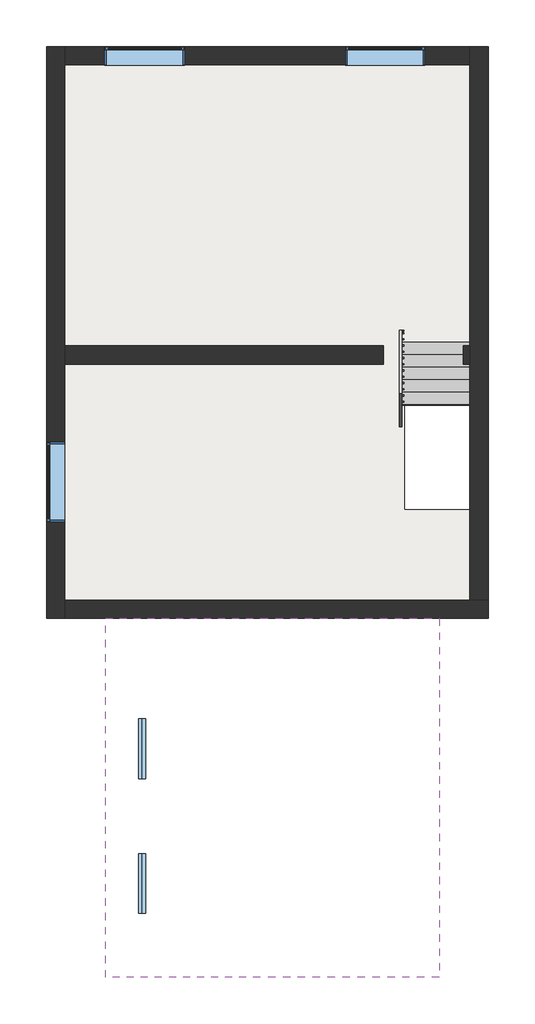
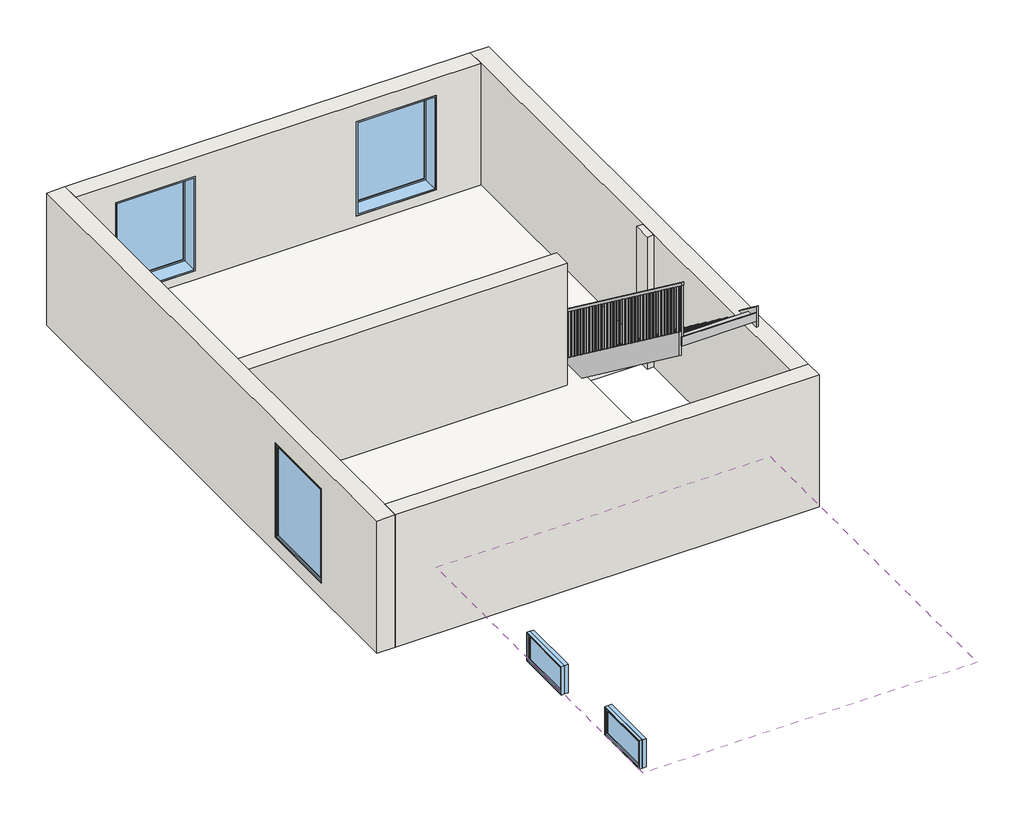
# One storey: 5 walls, 5 windows, 2 members, 1 railing, 1 roof, 1 slab, 1 stair flight.
"""IFC4 building model written with IfcOpenShell, lengths in millimetres."""

import ifcopenshell
import ifcopenshell.guid

model = None  # the IFC model being written
_history = None  # IfcOwnerHistory: only IFC2X3 demands one
_inside = {}  # id of a spatial element -> (the spatial element, [elements in it])
_under = {}  # id of a project, library or spatial element -> (it, [spatial elements below it])
_declared = {}  # id of a project -> (the project, [libraries it declares])
_typed = {}  # id of a type object -> (the type object, [elements of that type])
_made_of = {}  # id of a material, layer set ... -> (it, [elements and type objects made of it])


def new_model(schema):
    """Start an empty IFC model of exactly this schema.

    Asked for "IFC4X3", IfcOpenShell would pick the latest addendum, in which some entities
    have other attributes; the version numbers below select the first issue.
    IFC2X3 requires an IfcOwnerHistory on every rooted entity: one is made here for all.
    """
    global model, _history
    if schema == "IFC4X3":
        model = ifcopenshell.file(schema_version=(4, 3, 0, 0))
    else:
        model = ifcopenshell.file(schema=schema)
    _inside.clear()
    _under.clear()
    _declared.clear()
    _typed.clear()
    _made_of.clear()
    _history = None
    if model.schema == "IFC2X3":
        org = make("IfcOrganization", Name="unknown")
        user = make(
            "IfcPersonAndOrganization",
            ThePerson=make("IfcPerson", FamilyName="unknown"),
            TheOrganization=org,
        )
        app = make(
            "IfcApplication",
            ApplicationDeveloper=org,
            Version="unknown",
            ApplicationFullName="unknown",
            ApplicationIdentifier="unknown",
        )
        _history = make(
            "IfcOwnerHistory",
            OwningUser=user,
            OwningApplication=app,
            ChangeAction="ADDED",
            CreationDate=0,
        )
    return model


def make(cls, **values):
    """One entity of the class cls with the attributes given. An attribute that is None is left unset."""
    return model.create_entity(
        cls, **{name: value for name, value in values.items() if value is not None}
    )


def rooted(cls, **values):
    """An entity with a GlobalId (a new one), such as an element, a storey or a relation."""
    return make(cls, GlobalId=ifcopenshell.guid.new(), OwnerHistory=_history, **values)


def si_unit(unit_type, name, prefix=None):
    """IfcSIUnit, for example si_unit("LENGTHUNIT", "METRE", prefix="MILLI")."""
    return make("IfcSIUnit", UnitType=unit_type, Prefix=prefix, Name=name)


def assignment(units):
    """IfcUnitAssignment: the units of a project."""
    return None if units is None else make("IfcUnitAssignment", Units=units)


def point(xyz):
    """IfcCartesianPoint."""
    return None if xyz is None else make("IfcCartesianPoint", Coordinates=xyz)


def direction(xyz):
    """IfcDirection."""
    return None if xyz is None else make("IfcDirection", DirectionRatios=xyz)


def frame(location, z_axis=None, x_axis=None):
    """IfcAxis2Placement3D, a coordinate frame: its origin and axes. An axis left out is left unset."""
    return make(
        "IfcAxis2Placement3D",
        Location=point(location),
        Axis=direction(z_axis),
        RefDirection=direction(x_axis),
    )


def origin():
    """The frame at (0, 0, 0) with its axes left unset."""
    return frame((0.0, 0.0, 0.0))


def place(relative_to, where):
    """IfcLocalPlacement: puts the frame where relative to a parent placement (None: the world)."""
    return make(
        "IfcLocalPlacement", PlacementRelTo=relative_to, RelativePlacement=where
    )


def context(
    kind, dimensions, precision=None, world=None, true_north=None, identifier=None
):
    """IfcGeometricRepresentationContext, for example the 3D "Model" context."""
    return make(
        "IfcGeometricRepresentationContext",
        ContextIdentifier=identifier,
        ContextType=kind,
        CoordinateSpaceDimension=dimensions,
        Precision=precision,
        WorldCoordinateSystem=world,
        TrueNorth=true_north,
    )


def project(units=None, contexts=None):
    """IfcProject with its units and contexts."""
    return rooted(
        "IfcProject",
        Name="project",
        RepresentationContexts=contexts,
        UnitsInContext=assignment(units),
    )


def spatial(cls, under=None, at=None, **own):
    """A site, building, storey or space (cls), placed at a placement, below another one or the project."""
    s = rooted(cls, ObjectPlacement=at, **own)
    if under is not None:
        _under.setdefault(under.id(), (under, []))[1].append(s)
    return s


def polyline(points):
    """IfcPolyline through the points."""
    return make("IfcPolyline", Points=[point(p) for p in points])


def outline(outer, holes=None, kind="AREA"):
    """IfcArbitraryClosedProfileDef: a profile drawn as a closed curve; with holes, ...WithVoids."""
    if holes is None:
        return make("IfcArbitraryClosedProfileDef", ProfileType=kind, OuterCurve=outer)
    return make(
        "IfcArbitraryProfileDefWithVoids",
        ProfileType=kind,
        OuterCurve=outer,
        InnerCurves=holes,
    )


def extrude(swept, where, along, depth):
    """IfcExtrudedAreaSolid: the profile swept, set in the frame where, extruded along a direction by depth."""
    return make(
        "IfcExtrudedAreaSolid",
        SweptArea=swept,
        Position=where,
        ExtrudedDirection=direction(along),
        Depth=depth,
    )


def faces_of(points, faces, orient=None, outer=None):
    """IfcFace entities. A face is a list of loops; a loop is a list of indices into points, from 0.

    orient and outer hold one flag for each loop. By default every Orientation is true, the
    first loop of a face is its IfcFaceOuterBound and the others are IfcFaceBound.
    """
    made = []
    for i, loops in enumerate(faces):
        bounds = []
        for j, loop in enumerate(loops):
            is_outer = j == 0 if outer is None else outer[i][j]
            bounds.append(
                make(
                    "IfcFaceOuterBound" if is_outer else "IfcFaceBound",
                    Bound=make("IfcPolyLoop", Polygon=[points[k] for k in loop]),
                    Orientation=True if orient is None else orient[i][j],
                )
            )
        made.append(make("IfcFace", Bounds=bounds))
    return made


def faceted_brep(points, faces, orient=None, outer=None, voids=None):
    """IfcFacetedBrep: a solid bounded by flat faces; with voids (closed shells), ...WithVoids."""
    shared = [point(p) for p in points]
    hull = make("IfcClosedShell", CfsFaces=faces_of(shared, faces, orient, outer))
    if voids is None:
        return make("IfcFacetedBrep", Outer=hull)
    return make(
        "IfcFacetedBrepWithVoids",
        Outer=hull,
        Voids=[
            make(cls, CfsFaces=faces_of(shared, fs, o, b)) for cls, fs, o, b in voids
        ],
    )


def shape(context_of_items, identifier, shape_type, items):
    """IfcShapeRepresentation: the items that make up one representation, for example the "Body"."""
    return make(
        "IfcShapeRepresentation",
        ContextOfItems=context_of_items,
        RepresentationIdentifier=identifier,
        RepresentationType=shape_type,
        Items=items,
    )


def source(mapping_origin, context_of_items, identifier, shape_type, items):
    """IfcRepresentationMap: a shape defined once, which mapped items show again and again."""
    return make(
        "IfcRepresentationMap",
        MappingOrigin=mapping_origin,
        MappedRepresentation=shape(context_of_items, identifier, shape_type, items),
    )


def transform(
    local_origin,
    x_axis=None,
    y_axis=None,
    z_axis=None,
    scale=None,
    scale2=None,
    scale3=None,
    uniform=True,
):
    """IfcCartesianTransformationOperator3D, or its non-uniform kind. x_axis, y_axis, z_axis: its Axis1, 2, 3."""
    if uniform:
        return make(
            "IfcCartesianTransformationOperator3D",
            Axis1=direction(x_axis),
            Axis2=direction(y_axis),
            LocalOrigin=point(local_origin),
            Scale=scale,
            Axis3=direction(z_axis),
        )
    return make(
        "IfcCartesianTransformationOperator3DnonUniform",
        Axis1=direction(x_axis),
        Axis2=direction(y_axis),
        LocalOrigin=point(local_origin),
        Scale=scale,
        Axis3=direction(z_axis),
        Scale2=scale2,
        Scale3=scale3,
    )


def mapped(mapping_source, mapping_target):
    """IfcMappedItem: shows the shape of a source again, moved by a transform."""
    return make(
        "IfcMappedItem", MappingSource=mapping_source, MappingTarget=mapping_target
    )


def made_of(thing, what):
    """Note that an element or type object is made of a material, layer set ...; save() writes the relation."""
    if what is not None:
        _made_of.setdefault(what.id(), (what, []))[1].append(thing)
    return thing


def element(
    cls,
    number,
    at=None,
    inside=None,
    cuts=None,
    type_object=None,
    material=None,
    context=None,
    identifier="Body",
    shape_type=None,
    held_by="IfcProductDefinitionShape",
    body=None,
    shapes=None,
    **own,
):
    """One element of the class cls, such as IfcWall. Its Tag is "e" and its number.

    at: its placement. inside: the storey or other place that contains it. cuts: it is an
    opening in that element (IfcRelVoidsElement). A single representation is given by context,
    identifier, shape_type and body (its items); several are given by shapes. held_by: the class
    of the entity that holds the representations. save() writes the other relations.
    """
    e = rooted(cls, Tag="e%d" % number, ObjectPlacement=at, **own)
    if body is not None:
        shapes = [shape(context, identifier, shape_type, body)]
    if shapes is not None:
        e.Representation = make(held_by, Representations=shapes)
    if inside is not None:
        _inside.setdefault(inside.id(), (inside, []))[1].append(e)
    if cuts is not None:
        rooted(
            "IfcRelVoidsElement", RelatingBuildingElement=cuts, RelatedOpeningElement=e
        )
    if type_object is not None:
        _typed.setdefault(type_object.id(), (type_object, []))[1].append(e)
    return made_of(e, material)


def aggregate(whole, parts):
    """IfcRelAggregates: a whole, such as a stair, and the parts it consists of."""
    return rooted("IfcRelAggregates", RelatingObject=whole, RelatedObjects=parts)


def save(model, path):
    """Write the relations noted so far, then the file.

    IfcRelAggregates (storeys below a building ...), IfcRelContainedInSpatialStructure (elements
    in a storey), IfcRelDefinesByType, IfcRelAssociatesMaterial and IfcRelDeclares: one each for
    every whole, place, type object, material and project.
    """
    for whole, parts in _under.values():
        aggregate(whole, parts)
    for where, things in _inside.values():
        rooted(
            "IfcRelContainedInSpatialStructure",
            RelatedElements=things,
            RelatingStructure=where,
        )
    for kind, things in _typed.values():
        rooted("IfcRelDefinesByType", RelatedObjects=things, RelatingType=kind)
    for what, things in _made_of.values():
        rooted("IfcRelAssociatesMaterial", RelatedObjects=things, RelatingMaterial=what)
    for by, libraries in _declared.values():
        rooted("IfcRelDeclares", RelatingContext=by, RelatedDefinitions=libraries)
    model.write(path)


def stair_flight_c9982ff6(model_context):
    return source(origin(), model_context, "Body", "SweptSolid", [
        extrude(outline(polyline([(-11930.6631644, -7734.8774925), (-11930.6631644, -7722.3774925), (-10430.6631644, -7722.3774925), (-10430.6631644, -7734.8774925), (-11930.6631644, -7734.8774925)])), frame((0.0, 0.0, 2800.0), z_axis=(0.0, 0.0, 1.0), x_axis=(1.0, 0.0, 0.0)), (0.0, 0.0, 1.0), 136.6666667),
        extrude(outline(polyline([(-10430.6631644, -7972.3774925), (-11930.6631644, -7972.3774925), (-11930.6631644, -7722.3774925), (-10430.6631644, -7722.3774925), (-10430.6631644, -7972.3774925)])), frame((0.0, 0.0, 2936.6666667), z_axis=(0.0, 0.0, 1.0), x_axis=(1.0, 0.0, 0.0)), (0.0, 0.0, 1.0), 50.0),
        extrude(outline(polyline([(-11930.6631644, -7984.8774925), (-11930.6631644, -7972.3774925), (-10430.6631644, -7972.3774925), (-10430.6631644, -7984.8774925), (-11930.6631644, -7984.8774925)])), frame((0.0, 0.0, 2936.6666667), z_axis=(0.0, 0.0, 1.0), x_axis=(1.0, 0.0, 0.0)), (0.0, 0.0, 1.0), 186.6666667),
        extrude(outline(polyline([(-10430.6631644, -8222.3774925), (-11930.6631644, -8222.3774925), (-11930.6631644, -7972.3774925), (-10430.6631644, -7972.3774925), (-10430.6631644, -8222.3774925)])), frame((0.0, 0.0, 3123.3333333), z_axis=(0.0, 0.0, 1.0), x_axis=(1.0, 0.0, 0.0)), (0.0, 0.0, 1.0), 50.0),
        extrude(outline(polyline([(-11930.6631644, -8234.8774925), (-11930.6631644, -8222.3774925), (-10430.6631644, -8222.3774925), (-10430.6631644, -8234.8774925), (-11930.6631644, -8234.8774925)])), frame((0.0, 0.0, 3123.3333333), z_axis=(0.0, 0.0, 1.0), x_axis=(1.0, 0.0, 0.0)), (0.0, 0.0, 1.0), 186.6666667),
        extrude(outline(polyline([(-10430.6631644, -8472.3774925), (-11930.6631644, -8472.3774925), (-11930.6631644, -8222.3774925), (-10430.6631644, -8222.3774925), (-10430.6631644, -8472.3774925)])), frame((0.0, 0.0, 3310.0), z_axis=(0.0, 0.0, 1.0), x_axis=(1.0, 0.0, 0.0)), (0.0, 0.0, 1.0), 50.0),
        extrude(outline(polyline([(-11930.6631644, -8484.8774925), (-11930.6631644, -8472.3774925), (-10430.6631644, -8472.3774925), (-10430.6631644, -8484.8774925), (-11930.6631644, -8484.8774925)])), frame((0.0, 0.0, 3310.0), z_axis=(0.0, 0.0, 1.0), x_axis=(1.0, 0.0, 0.0)), (0.0, 0.0, 1.0), 186.6666667),
        extrude(outline(polyline([(-10430.6631644, -8722.3774925), (-11930.6631644, -8722.3774925), (-11930.6631644, -8472.3774925), (-10430.6631644, -8472.3774925), (-10430.6631644, -8722.3774925)])), frame((0.0, 0.0, 3496.6666667), z_axis=(0.0, 0.0, 1.0), x_axis=(1.0, 0.0, 0.0)), (0.0, 0.0, 1.0), 50.0),
        extrude(outline(polyline([(-11930.6631644, -8734.8774925), (-11930.6631644, -8722.3774925), (-10430.6631644, -8722.3774925), (-10430.6631644, -8734.8774925), (-11930.6631644, -8734.8774925)])), frame((0.0, 0.0, 3496.6666667), z_axis=(0.0, 0.0, 1.0), x_axis=(1.0, 0.0, 0.0)), (0.0, 0.0, 1.0), 186.6666667),
        extrude(outline(polyline([(-10430.6631644, -8972.3774925), (-11930.6631644, -8972.3774925), (-11930.6631644, -8722.3774925), (-10430.6631644, -8722.3774925), (-10430.6631644, -8972.3774925)])), frame((0.0, 0.0, 3683.3333333), z_axis=(0.0, 0.0, 1.0), x_axis=(1.0, 0.0, 0.0)), (0.0, 0.0, 1.0), 50.0),
        extrude(outline(polyline([(-11930.6631644, -8984.8774925), (-11930.6631644, -8972.3774925), (-10430.6631644, -8972.3774925), (-10430.6631644, -8984.8774925), (-11930.6631644, -8984.8774925)])), frame((0.0, 0.0, 3683.3333333), z_axis=(0.0, 0.0, 1.0), x_axis=(1.0, 0.0, 0.0)), (0.0, 0.0, 1.0), 186.6666667),
        extrude(outline(polyline([(-10430.6631644, -9222.3774925), (-11930.6631644, -9222.3774925), (-11930.6631644, -8972.3774925), (-10430.6631644, -8972.3774925), (-10430.6631644, -9222.3774925)])), frame((0.0, 0.0, 3870.0), z_axis=(0.0, 0.0, 1.0), x_axis=(1.0, 0.0, 0.0)), (0.0, 0.0, 1.0), 50.0),
        extrude(outline(polyline([(-11930.6631644, -9234.8774925), (-11930.6631644, -9222.3774925), (-10430.6631644, -9222.3774925), (-10430.6631644, -9234.8774925), (-11930.6631644, -9234.8774925)])), frame((0.0, 0.0, 3870.0), z_axis=(0.0, 0.0, 1.0), x_axis=(1.0, 0.0, 0.0)), (0.0, 0.0, 1.0), 186.6666667),
        extrude(outline(polyline([(-10430.6631644, -9472.3774925), (-11930.6631644, -9472.3774925), (-11930.6631644, -9222.3774925), (-10430.6631644, -9222.3774925), (-10430.6631644, -9472.3774925)])), frame((0.0, 0.0, 4056.6666667), z_axis=(0.0, 0.0, 1.0), x_axis=(1.0, 0.0, 0.0)), (0.0, 0.0, 1.0), 50.0),
        extrude(outline(polyline([(-11930.6631644, -9484.8774925), (-11930.6631644, -9472.3774925), (-10430.6631644, -9472.3774925), (-10430.6631644, -9484.8774925), (-11930.6631644, -9484.8774925)])), frame((0.0, 0.0, 4056.6666667), z_axis=(0.0, 0.0, 1.0), x_axis=(1.0, 0.0, 0.0)), (0.0, 0.0, 1.0), 186.6666667),
        extrude(outline(polyline([(-10430.6631644, -9722.3774925), (-11930.6631644, -9722.3774925), (-11930.6631644, -9472.3774925), (-10430.6631644, -9472.3774925), (-10430.6631644, -9722.3774925)])), frame((0.0, 0.0, 4243.3333333), z_axis=(0.0, 0.0, 1.0), x_axis=(1.0, 0.0, 0.0)), (0.0, 0.0, 1.0), 50.0),
        extrude(outline(polyline([(-11930.6631644, -9734.8774925), (-11930.6631644, -9722.3774925), (-10430.6631644, -9722.3774925), (-10430.6631644, -9734.8774925), (-11930.6631644, -9734.8774925)])), frame((0.0, 0.0, 4243.3333333), z_axis=(0.0, 0.0, 1.0), x_axis=(1.0, 0.0, 0.0)), (0.0, 0.0, 1.0), 186.6666667),
        extrude(outline(polyline([(-10430.6631644, -9972.3774925), (-11930.6631644, -9972.3774925), (-11930.6631644, -9722.3774925), (-10430.6631644, -9722.3774925), (-10430.6631644, -9972.3774925)])), frame((0.0, 0.0, 4430.0), z_axis=(0.0, 0.0, 1.0), x_axis=(1.0, 0.0, 0.0)), (0.0, 0.0, 1.0), 50.0),
        extrude(outline(polyline([(-11930.6631644, -9984.8774925), (-11930.6631644, -9972.3774925), (-10430.6631644, -9972.3774925), (-10430.6631644, -9984.8774925), (-11930.6631644, -9984.8774925)])), frame((0.0, 0.0, 4430.0), z_axis=(0.0, 0.0, 1.0), x_axis=(1.0, 0.0, 0.0)), (0.0, 0.0, 1.0), 186.6666667),
        extrude(outline(polyline([(-10430.6631644, -10222.3774925), (-11930.6631644, -10222.3774925), (-11930.6631644, -9972.3774925), (-10430.6631644, -9972.3774925), (-10430.6631644, -10222.3774925)])), frame((0.0, 0.0, 4616.6666667), z_axis=(0.0, 0.0, 1.0), x_axis=(1.0, 0.0, 0.0)), (0.0, 0.0, 1.0), 50.0),
        extrude(outline(polyline([(-11930.6631644, -10234.8774925), (-11930.6631644, -10222.3774925), (-10430.6631644, -10222.3774925), (-10430.6631644, -10234.8774925), (-11930.6631644, -10234.8774925)])), frame((0.0, 0.0, 4616.6666667), z_axis=(0.0, 0.0, 1.0), x_axis=(1.0, 0.0, 0.0)), (0.0, 0.0, 1.0), 186.6666667),
        extrude(outline(polyline([(-10430.6631644, -10472.3774925), (-11930.6631644, -10472.3774925), (-11930.6631644, -10222.3774925), (-10430.6631644, -10222.3774925), (-10430.6631644, -10472.3774925)])), frame((0.0, 0.0, 4803.3333333), z_axis=(0.0, 0.0, 1.0), x_axis=(1.0, 0.0, 0.0)), (0.0, 0.0, 1.0), 50.0),
        extrude(outline(polyline([(-11930.6631644, -10484.8774925), (-11930.6631644, -10472.3774925), (-10430.6631644, -10472.3774925), (-10430.6631644, -10484.8774925), (-11930.6631644, -10484.8774925)])), frame((0.0, 0.0, 4803.3333333), z_axis=(0.0, 0.0, 1.0), x_axis=(1.0, 0.0, 0.0)), (0.0, 0.0, 1.0), 186.6666667),
        extrude(outline(polyline([(-10430.6631644, -10722.3774925), (-11930.6631644, -10722.3774925), (-11930.6631644, -10472.3774925), (-10430.6631644, -10472.3774925), (-10430.6631644, -10722.3774925)])), frame((0.0, 0.0, 4990.0), z_axis=(0.0, 0.0, 1.0), x_axis=(1.0, 0.0, 0.0)), (0.0, 0.0, 1.0), 50.0),
        extrude(outline(polyline([(-11930.6631644, -10734.8774925), (-11930.6631644, -10722.3774925), (-10430.6631644, -10722.3774925), (-10430.6631644, -10734.8774925), (-11930.6631644, -10734.8774925)])), frame((0.0, 0.0, 4990.0), z_axis=(0.0, 0.0, 1.0), x_axis=(1.0, 0.0, 0.0)), (0.0, 0.0, 1.0), 186.6666667),
        extrude(outline(polyline([(-10430.6631644, -10972.3774925), (-11930.6631644, -10972.3774925), (-11930.6631644, -10722.3774925), (-10430.6631644, -10722.3774925), (-10430.6631644, -10972.3774925)])), frame((0.0, 0.0, 5176.6666667), z_axis=(0.0, 0.0, 1.0), x_axis=(1.0, 0.0, 0.0)), (0.0, 0.0, 1.0), 50.0),
        extrude(outline(polyline([(-11930.6631644, -10984.8774925), (-11930.6631644, -10972.3774925), (-10430.6631644, -10972.3774925), (-10430.6631644, -10984.8774925), (-11930.6631644, -10984.8774925)])), frame((0.0, 0.0, 5176.6666667), z_axis=(0.0, 0.0, 1.0), x_axis=(1.0, 0.0, 0.0)), (0.0, 0.0, 1.0), 186.6666667),
        extrude(outline(polyline([(-10430.6631644, -11222.3774925), (-11930.6631644, -11222.3774925), (-11930.6631644, -10972.3774925), (-10430.6631644, -10972.3774925), (-10430.6631644, -11222.3774925)])), frame((0.0, 0.0, 5363.3333333), z_axis=(0.0, 0.0, 1.0), x_axis=(1.0, 0.0, 0.0)), (0.0, 0.0, 1.0), 50.0),
        extrude(outline(polyline([(-11930.6631644, -11234.8774925), (-11930.6631644, -11222.3774925), (-10430.6631644, -11222.3774925), (-10430.6631644, -11234.8774925), (-11930.6631644, -11234.8774925)])), frame((0.0, 0.0, 5363.3333333), z_axis=(0.0, 0.0, 1.0), x_axis=(1.0, 0.0, 0.0)), (0.0, 0.0, 1.0), 186.6666667),
        extrude(outline(polyline([(-10430.6631644, -11472.3774925), (-11930.6631644, -11472.3774925), (-11930.6631644, -11222.3774925), (-10430.6631644, -11222.3774925), (-10430.6631644, -11472.3774925)])), frame((0.0, 0.0, 5550.0), z_axis=(0.0, 0.0, 1.0), x_axis=(1.0, 0.0, 0.0)), (0.0, 0.0, 1.0), 50.0),
        extrude(outline(polyline([(-11930.6631644, -11484.8774925), (-11930.6631644, -11472.3774925), (-10430.6631644, -11472.3774925), (-10430.6631644, -11484.8774925), (-11930.6631644, -11484.8774925)])), frame((0.0, 0.0, 5550.0), z_axis=(0.0, 0.0, 1.0), x_axis=(1.0, 0.0, 0.0)), (0.0, 0.0, 1.0), 186.6666667),
        extrude(outline(polyline([(-10430.6631644, -11722.3774925), (-11930.6631644, -11722.3774925), (-11930.6631644, -11472.3774925), (-10430.6631644, -11472.3774925), (-10430.6631644, -11722.3774925)])), frame((0.0, 0.0, 5736.6666667), z_axis=(0.0, 0.0, 1.0), x_axis=(1.0, 0.0, 0.0)), (0.0, 0.0, 1.0), 50.0),
        extrude(outline(polyline([(-11930.6631644, -11734.8774925), (-11930.6631644, -11722.3774925), (-10430.6631644, -11722.3774925), (-10430.6631644, -11734.8774925), (-11930.6631644, -11734.8774925)])), frame((0.0, 0.0, 5736.6666667), z_axis=(0.0, 0.0, 1.0), x_axis=(1.0, 0.0, 0.0)), (0.0, 0.0, 1.0), 186.6666667),
    ])


def window_c2055f4e(model_context):
    return source(origin(), model_context, "Body", "SweptSolid", [
        extrude(outline(polyline([(-737.0, 163.0), (737.0, 163.0), (737.0, 151.0), (-737.0, 151.0), (-737.0, 163.0)])), frame((0.0, 0.0, 978.0), z_axis=(0.0, 0.0, 1.0), x_axis=(1.0, 0.0, 0.0)), (0.0, 0.0, 1.0), 1874.0),
        extrude(outline(polyline([(2896.0, -781.0), (934.0, -781.0), (934.0, 781.0), (2896.0, 781.0), (2896.0, -781.0)]), holes=[polyline([(2852.0, -737.0), (2852.0, 737.0), (978.0, 737.0), (978.0, -737.0), (2852.0, -737.0)])]), frame((0.0, 135.0, 0.0), z_axis=(0.0, 1.0, 0.0), x_axis=(0.0, 0.0, 1.0)), (0.0, 0.0, 1.0), 44.0),
        extrude(outline(polyline([(2915.0, -800.0), (915.0, -800.0), (915.0, 800.0), (2915.0, 800.0), (2915.0, -800.0)]), holes=[polyline([(2896.0, -781.0), (2896.0, 781.0), (934.0, 781.0), (934.0, -781.0), (2896.0, -781.0)])]), frame((0.0, 135.0, 0.0), z_axis=(0.0, 1.0, 0.0), x_axis=(0.0, 0.0, 1.0)), (0.0, 0.0, 1.0), 63.0),
        extrude(outline(polyline([(2915.0, -800.0), (915.0, -800.0), (915.0, 800.0), (2915.0, 800.0), (2915.0, -800.0)]), holes=[polyline([(2883.0, -768.0), (2883.0, 768.0), (947.0, 768.0), (947.0, -768.0), (2883.0, -768.0)])]), frame((0.0, -172.0, 0.0), z_axis=(0.0, 1.0, 0.0), x_axis=(0.0, 0.0, 1.0)), (0.0, 0.0, 1.0), 307.0),
    ])


def window_76e8b9e6(model_context):
    return source(origin(), model_context, "Body", "SweptSolid", [
        extrude(outline(polyline([(-537.0, 48.0), (537.0, 48.0), (537.0, 36.0), (-537.0, 36.0), (-537.0, 48.0)])), frame((0.0, 0.0, 978.0), z_axis=(0.0, 0.0, 1.0), x_axis=(1.0, 0.0, 0.0)), (0.0, 0.0, 1.0), 474.0),
        extrude(outline(polyline([(1496.0, -581.0), (934.0, -581.0), (934.0, 581.0), (1496.0, 581.0), (1496.0, -581.0)]), holes=[polyline([(1452.0, -537.0), (1452.0, 537.0), (978.0, 537.0), (978.0, -537.0), (1452.0, -537.0)])]), frame((0.0, 20.0, 0.0), z_axis=(0.0, 1.0, 0.0), x_axis=(0.0, 0.0, 1.0)), (0.0, 0.0, 1.0), 44.0),
        extrude(outline(polyline([(1515.0, -600.0), (915.0, -600.0), (915.0, 600.0), (1515.0, 600.0), (1515.0, -600.0)]), holes=[polyline([(1496.0, -581.0), (1496.0, 581.0), (934.0, 581.0), (934.0, -581.0), (1496.0, -581.0)])]), frame((0.0, 20.0, 0.0), z_axis=(0.0, 1.0, 0.0), x_axis=(0.0, 0.0, 1.0)), (0.0, 0.0, 1.0), 63.0),
        extrude(outline(polyline([(1515.0, -600.0), (915.0, -600.0), (915.0, 600.0), (1515.0, 600.0), (1515.0, -600.0)]), holes=[polyline([(1483.0, -568.0), (1483.0, 568.0), (947.0, 568.0), (947.0, -568.0), (1483.0, -568.0)])]), frame((0.0, -57.0, 0.0), z_axis=(0.0, 1.0, 0.0), x_axis=(0.0, 0.0, 1.0)), (0.0, 0.0, 1.0), 77.0),
    ])


model = new_model("IFC4")

# Units and contexts
model_context = context("Model", 3, world=origin())
ifc_project = project(units=[si_unit("LENGTHUNIT", "METRE", prefix="MILLI")], contexts=[model_context])

# Site, building, storey
site = spatial("IfcSite", under=ifc_project)
building = spatial("IfcBuilding", under=site)
storey = spatial("IfcBuildingStorey", under=building, Name="Уровень 2", Elevation=2800.0)

# Members
placement = place(None, origin())
element("IfcMember", 1, ObjectType="Косоур/тетива - Ширина 50 мм", at=placement, inside=storey, context=model_context, shape_type="SweptSolid", body=[
    extrude(outline(polyline([(-7722.3774925, 3052.6673789), (-7722.3774925, 2800.0), (-8052.5566363, 2800.0), (-11722.3774925, 5540.132906), (-11722.3774925, 6039.3340456), (-7722.3774925, 3052.6673789)])), frame((-10430.6631644, 0.0, 0.0), z_axis=(1.0, 0.0, 0.0), x_axis=(0.0, 1.0, 0.0)), (0.0, 0.0, 1.0), 50.0),
])
element("IfcMember", 2, ObjectType="Косоур/тетива - Ширина 50 мм", at=placement, inside=storey, context=model_context, shape_type="SweptSolid", body=[
    extrude(outline(polyline([(-7722.3774925, 3052.6673789), (-7722.3774925, 2800.0), (-8052.5566363, 2800.0), (-11722.3774925, 5540.132906), (-11722.3774925, 6039.3340456), (-7722.3774925, 3052.6673789)])), frame((-11980.6631644, 0.0, 0.0), z_axis=(1.0, 0.0, 0.0), x_axis=(0.0, 1.0, 0.0)), (0.0, 0.0, 1.0), 50.0),
])

# Railing
element("IfcRailing", 3, ObjectType="1100 мм", at=placement, inside=storey, context=model_context, shape_type="SweptSolid", body=[
    extrude(outline(polyline([(-7722.3774925, 4086.6666667), (-7722.3774925, 4024.2665242), (-11722.3774925, 7010.9331909), (-11722.3774925, 7073.3333333), (-7722.3774925, 4086.6666667)])), frame((-11930.2631644, 0.0, 0.0), z_axis=(1.0, 0.0, 0.0), x_axis=(0.0, 1.0, 0.0)), (0.0, 0.0, 1.0), 50.0),
    extrude(outline(polyline([(-11647.3774925, 6954.9331909), (-11647.3774925, 5786.6666667), (-11672.3774925, 5786.6666667), (-11672.3774925, 6973.5998575), (-11647.3774925, 6954.9331909)])), frame((-11917.7631644, 0.0, 0.0), z_axis=(1.0, 0.0, 0.0), x_axis=(0.0, 1.0, 0.0)), (0.0, 0.0, 1.0), 25.0),
    extrude(outline(polyline([(-11522.3774925, 6861.5998575), (-11522.3774925, 5786.6666667), (-11547.3774925, 5786.6666667), (-11547.3774925, 6880.2665242), (-11522.3774925, 6861.5998575)])), frame((-11917.7631644, 0.0, 0.0), z_axis=(1.0, 0.0, 0.0), x_axis=(0.0, 1.0, 0.0)), (0.0, 0.0, 1.0), 25.0),
    extrude(outline(polyline([(-11397.3774925, 6768.2665242), (-11397.3774925, 5600.0), (-11422.3774925, 5600.0), (-11422.3774925, 6786.9331909), (-11397.3774925, 6768.2665242)])), frame((-11917.7631644, 0.0, 0.0), z_axis=(1.0, 0.0, 0.0), x_axis=(0.0, 1.0, 0.0)), (0.0, 0.0, 1.0), 25.0),
    extrude(outline(polyline([(-11272.3774925, 6674.9331909), (-11272.3774925, 5600.0), (-11297.3774925, 5600.0), (-11297.3774925, 6693.5998575), (-11272.3774925, 6674.9331909)])), frame((-11917.7631644, 0.0, 0.0), z_axis=(1.0, 0.0, 0.0), x_axis=(0.0, 1.0, 0.0)), (0.0, 0.0, 1.0), 25.0),
    extrude(outline(polyline([(-11147.3774925, 6581.5998575), (-11147.3774925, 5413.3333333), (-11172.3774925, 5413.3333333), (-11172.3774925, 6600.2665242), (-11147.3774925, 6581.5998575)])), frame((-11917.7631644, 0.0, 0.0), z_axis=(1.0, 0.0, 0.0), x_axis=(0.0, 1.0, 0.0)), (0.0, 0.0, 1.0), 25.0),
    extrude(outline(polyline([(-11022.3774925, 6488.2665242), (-11022.3774925, 5413.3333333), (-11047.3774925, 5413.3333333), (-11047.3774925, 6506.9331909), (-11022.3774925, 6488.2665242)])), frame((-11917.7631644, 0.0, 0.0), z_axis=(1.0, 0.0, 0.0), x_axis=(0.0, 1.0, 0.0)), (0.0, 0.0, 1.0), 25.0),
    extrude(outline(polyline([(-10897.3774925, 6394.9331909), (-10897.3774925, 5226.6666667), (-10922.3774925, 5226.6666667), (-10922.3774925, 6413.5998575), (-10897.3774925, 6394.9331909)])), frame((-11917.7631644, 0.0, 0.0), z_axis=(1.0, 0.0, 0.0), x_axis=(0.0, 1.0, 0.0)), (0.0, 0.0, 1.0), 25.0),
    extrude(outline(polyline([(-10772.3774925, 6301.5998575), (-10772.3774925, 5226.6666667), (-10797.3774925, 5226.6666667), (-10797.3774925, 6320.2665242), (-10772.3774925, 6301.5998575)])), frame((-11917.7631644, 0.0, 0.0), z_axis=(1.0, 0.0, 0.0), x_axis=(0.0, 1.0, 0.0)), (0.0, 0.0, 1.0), 25.0),
    extrude(outline(polyline([(-10647.3774925, 6208.2665242), (-10647.3774925, 5040.0), (-10672.3774925, 5040.0), (-10672.3774925, 6226.9331909), (-10647.3774925, 6208.2665242)])), frame((-11917.7631644, 0.0, 0.0), z_axis=(1.0, 0.0, 0.0), x_axis=(0.0, 1.0, 0.0)), (0.0, 0.0, 1.0), 25.0),
    extrude(outline(polyline([(-10522.3774925, 6114.9331909), (-10522.3774925, 5040.0), (-10547.3774925, 5040.0), (-10547.3774925, 6133.5998575), (-10522.3774925, 6114.9331909)])), frame((-11917.7631644, 0.0, 0.0), z_axis=(1.0, 0.0, 0.0), x_axis=(0.0, 1.0, 0.0)), (0.0, 0.0, 1.0), 25.0),
    extrude(outline(polyline([(-10397.3774925, 6021.5998575), (-10397.3774925, 4853.3333333), (-10422.3774925, 4853.3333333), (-10422.3774925, 6040.2665242), (-10397.3774925, 6021.5998575)])), frame((-11917.7631644, 0.0, 0.0), z_axis=(1.0, 0.0, 0.0), x_axis=(0.0, 1.0, 0.0)), (0.0, 0.0, 1.0), 25.0),
    extrude(outline(polyline([(-10272.3774925, 5928.2665242), (-10272.3774925, 4853.3333333), (-10297.3774925, 4853.3333333), (-10297.3774925, 5946.9331909), (-10272.3774925, 5928.2665242)])), frame((-11917.7631644, 0.0, 0.0), z_axis=(1.0, 0.0, 0.0), x_axis=(0.0, 1.0, 0.0)), (0.0, 0.0, 1.0), 25.0),
    extrude(outline(polyline([(-10147.3774925, 5834.9331909), (-10147.3774925, 4666.6666667), (-10172.3774925, 4666.6666667), (-10172.3774925, 5853.5998575), (-10147.3774925, 5834.9331909)])), frame((-11917.7631644, 0.0, 0.0), z_axis=(1.0, 0.0, 0.0), x_axis=(0.0, 1.0, 0.0)), (0.0, 0.0, 1.0), 25.0),
    extrude(outline(polyline([(-10022.3774925, 5741.5998575), (-10022.3774925, 4666.6666667), (-10047.3774925, 4666.6666667), (-10047.3774925, 5760.2665242), (-10022.3774925, 5741.5998575)])), frame((-11917.7631644, 0.0, 0.0), z_axis=(1.0, 0.0, 0.0), x_axis=(0.0, 1.0, 0.0)), (0.0, 0.0, 1.0), 25.0),
    extrude(outline(polyline([(-9897.3774925, 5648.2665242), (-9897.3774925, 4480.0), (-9922.3774925, 4480.0), (-9922.3774925, 5666.9331909), (-9897.3774925, 5648.2665242)])), frame((-11917.7631644, 0.0, 0.0), z_axis=(1.0, 0.0, 0.0), x_axis=(0.0, 1.0, 0.0)), (0.0, 0.0, 1.0), 25.0),
    extrude(outline(polyline([(-9772.3774925, 5554.9331909), (-9772.3774925, 4480.0), (-9797.3774925, 4480.0), (-9797.3774925, 5573.5998575), (-9772.3774925, 5554.9331909)])), frame((-11917.7631644, 0.0, 0.0), z_axis=(1.0, 0.0, 0.0), x_axis=(0.0, 1.0, 0.0)), (0.0, 0.0, 1.0), 25.0),
    extrude(outline(polyline([(-9647.3774925, 5461.5998575), (-9647.3774925, 4293.3333333), (-9672.3774925, 4293.3333333), (-9672.3774925, 5480.2665242), (-9647.3774925, 5461.5998575)])), frame((-11917.7631644, 0.0, 0.0), z_axis=(1.0, 0.0, 0.0), x_axis=(0.0, 1.0, 0.0)), (0.0, 0.0, 1.0), 25.0),
    extrude(outline(polyline([(-9522.3774925, 5368.2665242), (-9522.3774925, 4293.3333333), (-9547.3774925, 4293.3333333), (-9547.3774925, 5386.9331909), (-9522.3774925, 5368.2665242)])), frame((-11917.7631644, 0.0, 0.0), z_axis=(1.0, 0.0, 0.0), x_axis=(0.0, 1.0, 0.0)), (0.0, 0.0, 1.0), 25.0),
    extrude(outline(polyline([(-9397.3774925, 5274.9331909), (-9397.3774925, 4106.6666667), (-9422.3774925, 4106.6666667), (-9422.3774925, 5293.5998575), (-9397.3774925, 5274.9331909)])), frame((-11917.7631644, 0.0, 0.0), z_axis=(1.0, 0.0, 0.0), x_axis=(0.0, 1.0, 0.0)), (0.0, 0.0, 1.0), 25.0),
    extrude(outline(polyline([(-9272.3774925, 5181.5998575), (-9272.3774925, 4106.6666667), (-9297.3774925, 4106.6666667), (-9297.3774925, 5200.2665242), (-9272.3774925, 5181.5998575)])), frame((-11917.7631644, 0.0, 0.0), z_axis=(1.0, 0.0, 0.0), x_axis=(0.0, 1.0, 0.0)), (0.0, 0.0, 1.0), 25.0),
    extrude(outline(polyline([(-9147.3774925, 5088.2665242), (-9147.3774925, 3920.0), (-9172.3774925, 3920.0), (-9172.3774925, 5106.9331909), (-9147.3774925, 5088.2665242)])), frame((-11917.7631644, 0.0, 0.0), z_axis=(1.0, 0.0, 0.0), x_axis=(0.0, 1.0, 0.0)), (0.0, 0.0, 1.0), 25.0),
    extrude(outline(polyline([(-9022.3774925, 4994.9331909), (-9022.3774925, 3920.0), (-9047.3774925, 3920.0), (-9047.3774925, 5013.5998575), (-9022.3774925, 4994.9331909)])), frame((-11917.7631644, 0.0, 0.0), z_axis=(1.0, 0.0, 0.0), x_axis=(0.0, 1.0, 0.0)), (0.0, 0.0, 1.0), 25.0),
    extrude(outline(polyline([(-8897.3774925, 4901.5998575), (-8897.3774925, 3733.3333333), (-8922.3774925, 3733.3333333), (-8922.3774925, 4920.2665242), (-8897.3774925, 4901.5998575)])), frame((-11917.7631644, 0.0, 0.0), z_axis=(1.0, 0.0, 0.0), x_axis=(0.0, 1.0, 0.0)), (0.0, 0.0, 1.0), 25.0),
    extrude(outline(polyline([(-8772.3774925, 4808.2665242), (-8772.3774925, 3733.3333333), (-8797.3774925, 3733.3333333), (-8797.3774925, 4826.9331909), (-8772.3774925, 4808.2665242)])), frame((-11917.7631644, 0.0, 0.0), z_axis=(1.0, 0.0, 0.0), x_axis=(0.0, 1.0, 0.0)), (0.0, 0.0, 1.0), 25.0),
    extrude(outline(polyline([(-8647.3774925, 4714.9331909), (-8647.3774925, 3546.6666667), (-8672.3774925, 3546.6666667), (-8672.3774925, 4733.5998575), (-8647.3774925, 4714.9331909)])), frame((-11917.7631644, 0.0, 0.0), z_axis=(1.0, 0.0, 0.0), x_axis=(0.0, 1.0, 0.0)), (0.0, 0.0, 1.0), 25.0),
    extrude(outline(polyline([(-8522.3774925, 4621.5998575), (-8522.3774925, 3546.6666667), (-8547.3774925, 3546.6666667), (-8547.3774925, 4640.2665242), (-8522.3774925, 4621.5998575)])), frame((-11917.7631644, 0.0, 0.0), z_axis=(1.0, 0.0, 0.0), x_axis=(0.0, 1.0, 0.0)), (0.0, 0.0, 1.0), 25.0),
    extrude(outline(polyline([(-8397.3774925, 4528.2665242), (-8397.3774925, 3360.0), (-8422.3774925, 3360.0), (-8422.3774925, 4546.9331909), (-8397.3774925, 4528.2665242)])), frame((-11917.7631644, 0.0, 0.0), z_axis=(1.0, 0.0, 0.0), x_axis=(0.0, 1.0, 0.0)), (0.0, 0.0, 1.0), 25.0),
    extrude(outline(polyline([(-8272.3774925, 4434.9331909), (-8272.3774925, 3360.0), (-8297.3774925, 3360.0), (-8297.3774925, 4453.5998575), (-8272.3774925, 4434.9331909)])), frame((-11917.7631644, 0.0, 0.0), z_axis=(1.0, 0.0, 0.0), x_axis=(0.0, 1.0, 0.0)), (0.0, 0.0, 1.0), 25.0),
    extrude(outline(polyline([(-8147.3774925, 4341.5998575), (-8147.3774925, 3173.3333333), (-8172.3774925, 3173.3333333), (-8172.3774925, 4360.2665242), (-8147.3774925, 4341.5998575)])), frame((-11917.7631644, 0.0, 0.0), z_axis=(1.0, 0.0, 0.0), x_axis=(0.0, 1.0, 0.0)), (0.0, 0.0, 1.0), 25.0),
    extrude(outline(polyline([(-8022.3774925, 4248.2665242), (-8022.3774925, 3173.3333333), (-8047.3774925, 3173.3333333), (-8047.3774925, 4266.9331909), (-8022.3774925, 4248.2665242)])), frame((-11917.7631644, 0.0, 0.0), z_axis=(1.0, 0.0, 0.0), x_axis=(0.0, 1.0, 0.0)), (0.0, 0.0, 1.0), 25.0),
    extrude(outline(polyline([(-7897.3774925, 4154.9331909), (-7897.3774925, 2986.6666667), (-7922.3774925, 2986.6666667), (-7922.3774925, 4173.5998575), (-7897.3774925, 4154.9331909)])), frame((-11917.7631644, 0.0, 0.0), z_axis=(1.0, 0.0, 0.0), x_axis=(0.0, 1.0, 0.0)), (0.0, 0.0, 1.0), 25.0),
    extrude(outline(polyline([(-7772.3774925, 4061.5998575), (-7772.3774925, 2986.6666667), (-7797.3774925, 2986.6666667), (-7797.3774925, 4080.2665242), (-7772.3774925, 4061.5998575)])), frame((-11917.7631644, 0.0, 0.0), z_axis=(1.0, 0.0, 0.0), x_axis=(0.0, 1.0, 0.0)), (0.0, 0.0, 1.0), 25.0),
    extrude(outline(polyline([(-11697.3774925, 6992.2665242), (-11697.3774925, 5786.6666667), (-11722.3774925, 5786.6666667), (-11722.3774925, 7010.9331909), (-11697.3774925, 6992.2665242)])), frame((-11917.7631644, 0.0, 0.0), z_axis=(1.0, 0.0, 0.0), x_axis=(0.0, 1.0, 0.0)), (0.0, 0.0, 1.0), 25.0),
    extrude(outline(polyline([(-7722.3774925, 4024.2665242), (-7722.3774925, 2986.6666667), (-7747.3774925, 2986.6666667), (-7747.3774925, 4042.9331909), (-7722.3774925, 4024.2665242)])), frame((-11917.7631644, 0.0, 0.0), z_axis=(1.0, 0.0, 0.0), x_axis=(0.0, 1.0, 0.0)), (0.0, 0.0, 1.0), 25.0),
])

# Roof
element("IfcRoof", 4, ObjectType="Типовой - 125мм", at=placement, inside=storey, context=model_context, shape_type="SweptSolid", body=[
    extrude(outline(polyline([(4350.0, -11177.3789657), (6000.0, -14775.7187594), (4350.0, -17878.9174272), (4208.4287437, -17878.9174272), (5860.6067402, -14771.6225436), (4212.4850387, -11177.3789657), (4350.0, -11177.3789657)])), frame((0.0, -20707.3774925, 0.0), z_axis=(0.0, 1.0, 0.0), x_axis=(0.0, 0.0, 1.0)), (0.0, 0.0, 1.0), 7200.0),
])

# Slab
element("IfcSlab", 5, ObjectType="Фундаментная плита 220 мм", at=placement, inside=storey, context=model_context, shape_type="SweptSolid", body=[
    extrude(outline(polyline([(-10380.6631644, -2222.3774925), (-10380.6631644, -8222.3774925), (-11880.6631644, -8222.3774925), (-11880.6631644, -11322.3774925), (-10380.6631644, -11322.3774925), (-10380.6631644, -13322.3774925), (-11880.6631644, -13322.3774925), (-18880.6631644, -13322.3774925), (-18880.6631644, -2222.3774925), (-10380.6631644, -2222.3774925)])), frame((0.0, 0.0, 2800.0), z_axis=(0.0, 0.0, 1.0), x_axis=(1.0, 0.0, 0.0)), (0.0, 0.0, 1.0), 220.0),
])

# Stair flight
stair_flight_shape = stair_flight_c9982ff6(model_context)
element("IfcStairFlight", 6, ObjectType="Проступь 50 мм, подступенок 13 мм", at=placement, inside=storey, context=model_context, shape_type="MappedRepresentation", body=[
    mapped(stair_flight_shape, transform((0.0, 0.0, 0.0), x_axis=(1.0, 0.0, 0.0), y_axis=(0.0, 1.0, 0.0), z_axis=(0.0, 0.0, 1.0))),
])

# Walls
element("IfcWall", 7, ObjectType="Типовой - Кладка 370 мм", at=placement, inside=storey, context=model_context, shape_type="Brep", body=[
    faceted_brep([(-19065.6631644, -2037.3774925, 2800.0), (-19065.6631644, -13507.3774925, 2800.0), (-19065.6631644, -13507.3774925, 5600.0), (-19065.6631644, -2037.3774925, 5600.0), (-19065.6631644, -11572.3774925, 3113.5562909), (-19065.6631644, -9972.3774925, 3113.5562909), (-19065.6631644, -9972.3774925, 5113.5562909), (-19065.6631644, -11572.3774925, 5113.5562909), (-18695.6631644, -2037.3774925, 2800.0), (-18695.6631644, -2037.3774925, 5600.0), (-18695.6631644, -2407.3774925, 5600.0), (-18695.6631644, -8037.3774925, 5600.0), (-18695.6631644, -8407.3774925, 5600.0), (-18695.6631644, -13137.3774925, 5600.0), (-18695.6631644, -13507.3774925, 5600.0), (-18695.6631644, -13507.3774925, 2800.0), (-18695.6631644, -13137.3774925, 2800.0), (-18695.6631644, -8407.3774925, 2800.0), (-18695.6631644, -8037.3774925, 2800.0), (-18695.6631644, -2407.3774925, 2800.0), (-18695.6631644, -11572.3774925, 3113.5562909), (-18695.6631644, -11572.3774925, 5113.5562909), (-18695.6631644, -9972.3774925, 5113.5562909), (-18695.6631644, -9972.3774925, 3113.5562909)], [[[0, 1, 2, 3], [4, 5, 6, 7]], [[8, 9, 10, 11, 12, 13, 14, 15, 16, 17, 18, 19], [20, 21, 22, 23]], [[1, 0, 8, 19, 18, 17, 16, 15]], [[3, 2, 14, 13, 12, 11, 10, 9]], [[2, 1, 15, 14]], [[0, 3, 9, 8]], [[21, 20, 4, 7]], [[22, 21, 7, 6]], [[23, 22, 6, 5]], [[20, 23, 5, 4]]]),
])
element("IfcWall", 8, ObjectType="Типовой - Кладка 370 мм", at=placement, inside=storey, context=model_context, shape_type="Brep", body=[
    faceted_brep([(-18695.6631644, -13507.3774925, 2800.0), (-10195.6631644, -13507.3774925, 2800.0), (-10195.6631644, -13507.3774925, 5600.0), (-18695.6631644, -13507.3774925, 5600.0), (-18695.6631644, -13137.3774925, 2800.0), (-18695.6631644, -13137.3774925, 5600.0), (-10565.6631644, -13137.3774925, 5600.0), (-10195.6631644, -13137.3774925, 5600.0), (-10195.6631644, -13137.3774925, 2800.0), (-10565.6631644, -13137.3774925, 2800.0)], [[[0, 1, 2, 3]], [[4, 5, 6, 7, 8, 9]], [[1, 0, 4, 9, 8]], [[3, 2, 7, 6, 5]], [[0, 3, 5, 4]], [[2, 1, 8, 7]]]),
])
element("IfcWall", 9, ObjectType="Типовой - Кладка 370 мм", at=placement, inside=storey, context=model_context, shape_type="Brep", body=[
    faceted_brep([(-10195.6631644, -13137.3774925, 2800.0), (-10195.6631644, -2037.3774925, 2800.0), (-10195.6631644, -2037.3774925, 5600.0), (-10195.6631644, -13137.3774925, 5600.0), (-10565.6631644, -13137.3774925, 2800.0), (-10565.6631644, -13137.3774925, 5600.0), (-10565.6631644, -8407.3774925, 5600.0), (-10565.6631644, -8037.3774925, 5600.0), (-10565.6631644, -2407.3774925, 5600.0), (-10565.6631644, -2037.3774925, 5600.0), (-10565.6631644, -2037.3774925, 2800.0), (-10565.6631644, -2407.3774925, 2800.0), (-10565.6631644, -8037.3774925, 2800.0), (-10565.6631644, -8407.3774925, 2800.0)], [[[0, 1, 2, 3]], [[4, 5, 6, 7, 8, 9, 10, 11, 12, 13]], [[1, 0, 4, 13, 12, 11, 10]], [[3, 2, 9, 8, 7, 6, 5]], [[0, 3, 5, 4]], [[2, 1, 10, 9]]]),
])
element("IfcWall", 10, ObjectType="Типовой - Кладка 370 мм", at=placement, inside=storey, context=model_context, shape_type="SweptSolid", body=[
    extrude(outline(polyline([(2800.0, -10565.6631644), (5600.0, -10565.6631644), (5600.0, -18695.6631644), (2800.0, -18695.6631644), (2800.0, -10565.6631644)]), holes=[polyline([(3210.2974569, -17895.6631644), (5210.2974569, -17895.6631644), (5210.2974569, -16295.6631644), (3210.2974569, -16295.6631644), (3210.2974569, -17895.6631644)]), polyline([(3236.6142505, -13065.6631644), (5236.6142505, -13065.6631644), (5236.6142505, -11465.6631644), (3236.6142505, -11465.6631644), (3236.6142505, -13065.6631644)])]), frame((0.0, -2407.3774925, 0.0), z_axis=(0.0, 1.0, 0.0), x_axis=(0.0, 0.0, 1.0)), (0.0, 0.0, 1.0), 370.0),
])
element("IfcWall", 11, ObjectType="Типовой - Кладка 370 мм", at=placement, inside=storey, context=model_context, shape_type="SweptSolid", body=[
    extrude(outline(polyline([(-18695.6631644, -8407.3774925), (-18695.6631644, -8037.3774925), (-12298.8723784, -8037.3774925), (-12298.8723784, -8407.3774925), (-18695.6631644, -8407.3774925)])), frame((0.0, 0.0, 2800.0), z_axis=(0.0, 0.0, 1.0), x_axis=(1.0, 0.0, 0.0)), (0.0, 0.0, 1.0), 2800.0),
    extrude(outline(polyline([(-10565.6631644, -8037.3774925), (-10565.6631644, -8407.3774925), (-10698.8723784, -8407.3774925), (-10698.8723784, -8037.3774925), (-10565.6631644, -8037.3774925)])), frame((0.0, 0.0, 2800.0), z_axis=(0.0, 0.0, 1.0), x_axis=(1.0, 0.0, 0.0)), (0.0, 0.0, 1.0), 2800.0),
])

# Windows
window_shape = window_c2055f4e(model_context)
element("IfcWindow", 12, ObjectType="Фиксированные : 1600х2000", at=placement, inside=storey, context=model_context, shape_type="MappedRepresentation", body=[
    mapped(window_shape, transform((-17095.6631644, -2235.3774925, 2295.2974569), x_axis=(1.0, 0.0, 0.0), y_axis=(0.0, 1.0, 0.0), z_axis=(0.0, 0.0, 1.0))),
])
element("IfcWindow", 13, ObjectType="Фиксированные : 1600х2000", at=placement, inside=storey, context=model_context, shape_type="MappedRepresentation", body=[
    mapped(window_shape, transform((-12265.6631644, -2235.3774925, 2321.6142505), x_axis=(1.0, 0.0, 0.0), y_axis=(0.0, 1.0, 0.0), z_axis=(0.0, 0.0, 1.0))),
])
element("IfcWindow", 14, ObjectType="Фиксированные : 1600х2000", at=placement, inside=storey, context=model_context, shape_type="MappedRepresentation", body=[
    mapped(window_shape, transform((-18867.6631644, -10772.3774925, 2198.5562909), x_axis=(0.0, 1.0, 0.0), y_axis=(-1.0, 0.0, 0.0), z_axis=(0.0, 0.0, 1.0))),
])
window_2_shape = window_76e8b9e6(model_context)
element("IfcWindow", 15, ObjectType="Фиксированные : 1200х600", at=placement, inside=storey, context=model_context, shape_type="MappedRepresentation", body=[
    mapped(window_2_shape, transform((-17137.6631644, -18822.3774925, 2365.750298), x_axis=(0.0, 1.0, 0.0), y_axis=(-1.0, 0.0, 0.0), z_axis=(0.0, 0.0, 1.0))),
])
element("IfcWindow", 16, ObjectType="Фиксированные : 1200х600", at=placement, inside=storey, context=model_context, shape_type="MappedRepresentation", body=[
    mapped(window_2_shape, transform((-17137.6631644, -16122.3774925, 2301.8135789), x_axis=(0.0, 1.0, 0.0), y_axis=(-1.0, 0.0, 0.0), z_axis=(0.0, 0.0, 1.0))),
])

save(model, "model.ifc")

# Revit data of these elements
# Type "1100 мм"
#   built-in parameter 1008612 = 0.019685 (stored number, unit not read)
#   built-in parameter 1008611 = 0.019685 (stored number, unit not read)
#   built-in parameter 1008609 = 0.902231 (stored number, unit not read)
#   built-in parameter 1008604 = 0.19685 (stored number, unit not read)
#   built-in parameter 1008603 = 0.164042 (stored number, unit not read)
#   Railing Height = 1100 mm
#   built-in parameter 1008630 = 2
#   built-in parameter 1008610 = 2
#   built-in parameter 1008608 = 1
#   built-in parameter 1008618 = Балясина - Квадратная : 25  мм
# Type "Типовой - 125мм"
#   Layers, outside or top first: 125 mm no material (function 1)
# Type "Фундаментная плита 220 мм"
#   Layers, outside or top first: 220 mm "Бетон, монолитный" (function 1)
# Type "Типовой - Кладка 370 мм"
#   Layers, outside or top first: 370 mm "Бетонные модули для кладки" (function 1)
# Type "Фиксированные : 1600х2000"
#   Type Mark = "20"
#   Construction Type Id = "GSP4R"
#   Analytic Construction = "Одинарное остекление стеклами Пилкингтон - 1/8 дюйма"
#   Visual Light Transmittance = 0.9
#   Solar Heat Gain Coefficient = 0.78
#   Heat Transfer Coefficient (U) = 3.6886 W/(m²·K)
#   Height = 2000 mm
#   Высота подоконника по умолчанию = 915 mm
#   Width = 1600 mm
#   Вставка окна = 19 mm
#   Наружный материал каркаса = Переплет
#   Внутренний материал каркаса = Переплет
#   Материал оконного стекла = Стекло
#   Переплет = Переплет
#   Wall Closure = (empty or 0)
# Type "Фиксированные : 1200х600"
#   Type Mark = "19"
#   Construction Type Id = "GSP4R"
#   Analytic Construction = "Одинарное остекление стеклами Пилкингтон - 1/8 дюйма"
#   Visual Light Transmittance = 0.9
#   Solar Heat Gain Coefficient = 0.78
#   Heat Transfer Coefficient (U) = 3.6886 W/(m²·K)
#   Height = 600 mm
#   Высота подоконника по умолчанию = 915 mm
#   Width = 1200 mm
#   Вставка окна = 19 mm
#   Наружный материал каркаса = Переплет
#   Внутренний материал каркаса = Переплет
#   Материал оконного стекла = Стекло
#   Переплет = Переплет
#   Wall Closure = (empty or 0)
# Elements 1, 2 (IfcMember, "Косоур/тетива - Ширина 50 мм")
#   Phase Created = Новая конструкция
# Element 3 (IfcRailing, "1100 мм")
#   Phase Created = Новая конструкция
# Element 4 (IfcRoof, "Типовой - 125мм")
#   built-in parameter 1001710 = 33615
#   Phase Created = Новая конструкция
#   Materials on its faces: "Крыша по умолчанию"
# Element 5 (IfcSlab, "Фундаментная плита 220 мм")
#   Height Offset From Level = 220 mm
#   built-in parameter 1001954 = 1
#   Phase Created = Новая конструкция
#   Materials on its faces: "Бетон, монолитный"
# Element 6 (IfcStairFlight, "Проступь 50 мм, подступенок 13 мм")
#   Phase Created = Новая конструкция
# Elements 7, 8, 9, 10, 11 (IfcWall, "Типовой - Кладка 370 мм")
#   Comments = ""
#   Top Offset = 0 mm
#   Base Offset = 0 mm
#   Unconnected Height = 2800 mm
#   wall height = 2800 mm
#   Phase Created = Новая конструкция
#   Base Constraint = Уровень 2
#   Materials on its faces: "Бетонные модули для кладки"
# Element 12 (IfcWindow, "Фиксированные : 1600х2000")
#   Mark = "11"
#   Phase Created = Новая конструкция
#   Materials on its faces: "Переплет", "Стекло"
# Element 13 (IfcWindow, "Фиксированные : 1600х2000")
#   Mark = "12"
#   Phase Created = Новая конструкция
#   Materials on its faces: "Переплет", "Стекло"
# Element 14 (IfcWindow, "Фиксированные : 1600х2000")
#   Mark = "13"
#   Phase Created = Новая конструкция
#   Materials on its faces: "Переплет", "Стекло"
# Element 15 (IfcWindow, "Фиксированные : 1200х600")
#   Mark = "14"
#   Phase Created = Новая конструкция
#   Materials on its faces: "Переплет", "Стекло"
# Element 16 (IfcWindow, "Фиксированные : 1200х600")
#   Mark = "15"
#   Phase Created = Новая конструкция
#   Materials on its faces: "Переплет", "Стекло"
# Materials
#   "Бетон, монолитный": class "Бетон", colour RGB 192 192 192, transparency 0, Description = "физический материал", Cost = 0
#   "Бетонные модули для кладки": class "Кладка", colour RGB 181 181 181, transparency 0, Description = "Бетонные модули для кладки", Cost = 0
#   "Переплет": class "Древесина", colour RGB 224 178 126, transparency 0, Cost = 0
#   "Стекло": class "Стекло", colour RGB 0 128 192, transparency 0.9, Description = "Известково-натриевое стекло", Cost = 0
#   "Крыша по умолчанию": class "Разное", colour RGB 0 127 0, transparency 0, Cost = 0
